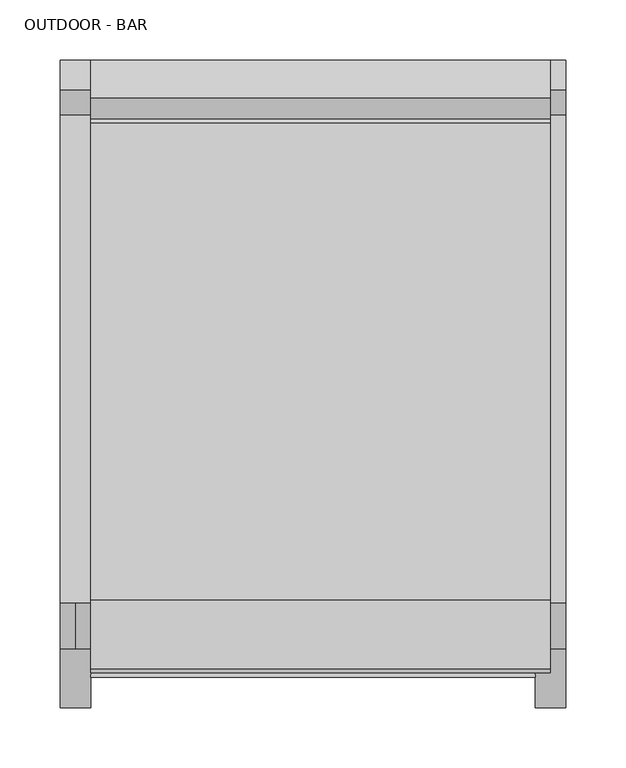
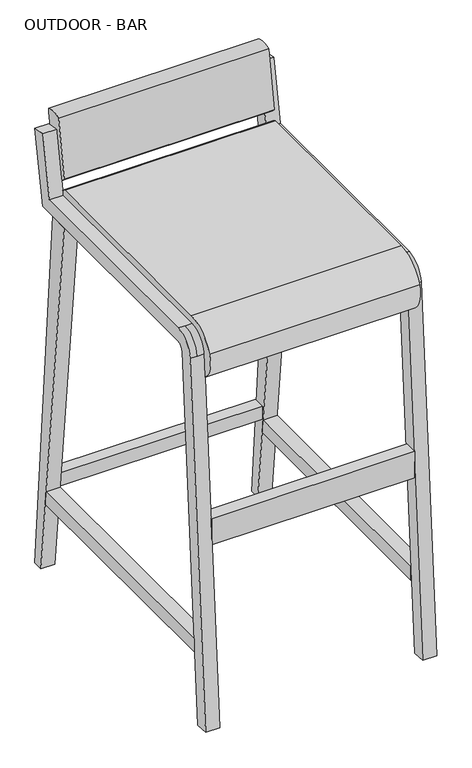
"""IFC4 building model written with IfcOpenShell, lengths in millimetres: furniture geometry, Bar_Stool_6722[1]1 : OUTDOOR - BAR."""

from ifc_helpers import new_model, si_unit, point, frame, frame_2d, origin, place, context, project, spatial, polyline, circle_curve, trimmed, segment, composite_curve, outline, extrude, source, transform, mapped, element, save
from ifc_brep_helpers import plane_surface, cylinder_surface, revolved_surface, advanced_brep


def outdoor_bar_9d95edac(model_context):
    return source(origin(), model_context, "Body", "SolidModel", [
        advanced_brep(
        [(419.1, -25.0141169, 838.4759165), (419.1, 0.0, 834.0652528), (393.7, 0.0, 834.0652528), (393.7, -25.0141169, 838.4759165), (393.7, -45.2169423, 723.9), (419.1, -45.2169423, 723.9), (393.7, -23.9038117, 698.5), (393.7, -450.0350637, 698.5), (393.7, -462.7032819, 686.6979128), (393.7, -511.439502, -0.8979128), (393.7, -536.7759384, 0.8979128), (393.7, -488.0397183, 688.4937383), (393.7, -450.0350637, 723.9), (419.1, -23.9038117, 698.5), (419.1, -450.0350637, 723.9), (419.1, -488.0397183, 688.4937383), (419.1, -536.7759384, 0.8979128), (419.1, -511.439502, -0.8979128), (419.1, -462.7032819, 686.6979128), (419.1, -450.0350637, 698.5), (406.4, -450.0350637, 723.9), (406.4, -488.0397183, 688.4937383)],
        [
            (0, 1),
            (1, 2),
            (2, 3),
            (3, 0),
            (3, 4),
            (4, 5),
            (5, 0),
            (2, 6),
            (6, 7),
            (7, 8, circle_curve(frame((393.7, -450.0350637, 685.8), z_axis=(1.0, 0.0, 0.0), x_axis=(0.0, 0.0, 1.0)), 12.7)),
            (8, 9),
            (9, 10),
            (10, 11),
            (11, 12, circle_curve(frame((393.7, -450.0350637, 685.8), z_axis=(-1.0, 0.0, 0.0), x_axis=(0.0, 0.0, 1.0)), 38.1)),
            (12, 4),
            (1, 13),
            (13, 6),
            (5, 14),
            (14, 15, circle_curve(frame((419.1, -450.0350637, 685.8), z_axis=(1.0, 0.0, 0.0), x_axis=(0.0, 0.0, 1.0)), 38.1)),
            (15, 16),
            (16, 17),
            (17, 18),
            (18, 19, circle_curve(frame((419.1, -450.0350637, 685.8), z_axis=(-1.0, 0.0, 0.0), x_axis=(0.0, 0.0, 1.0)), 12.7)),
            (19, 13),
            (12, 20),
            (20, 14),
            (19, 7),
            (21, 15),
            (20, 21, circle_curve(frame((406.4, -450.0350637, 685.8), z_axis=(1.0, 0.0, 0.0), x_axis=(0.0, 0.0, 1.0)), 38.1)),
            (11, 21),
            (18, 8),
            (10, 16),
            (17, 9),
        ],
        [
            plane_surface(frame((406.4, -12.5070585, 836.2705846), z_axis=(0.0, 0.17364817766692853, 0.9848077530122085), x_axis=(1.0, 0.0, 0.0))),
            plane_surface(frame((406.4, -25.0141169, 838.4759165), z_axis=(0.0, -0.9848077530122085, 0.17364817766692814), x_axis=(0.0, -0.17364817766692814, -0.9848077530122085))),
            plane_surface(frame((393.7, -25.0141169, 838.4759165), z_axis=(-1.0, 0.0, 0.0), x_axis=(0.0, -0.17364817766692808, -0.9848077530122085))),
            plane_surface(frame((393.7, 0.0, 834.0652528), z_axis=(0.0, 0.9848077530122085, -0.17364817766692817), x_axis=(0.0, -0.17364817766692817, -0.9848077530122085))),
            plane_surface(frame((419.1, 0.0, 834.0652528), z_axis=(1.0000000000000002, 0.0, 0.0), x_axis=(0.0, -0.1736481776669284, -0.9848077530122085))),
            plane_surface(frame((406.4, -45.2169423, 723.9), z_axis=(0.0, 0.0, 1.0), x_axis=(0.0, -1.0, 0.0))),
            plane_surface(frame((393.7, -23.9038117, 698.5), z_axis=(0.0, 0.0, -1.0), x_axis=(0.0, -1.0, 0.0))),
            cylinder_surface(frame((406.4, -450.0350637, 685.8), z_axis=(-1.0, 0.0, 0.0), x_axis=(0.0, 0.0, 1.0)), 38.1),
            revolved_surface(polyline([(393.7, -450.0350637, 698.5), (419.1, -450.0350637, 698.5)]), (406.4, -450.0350637, 685.8), (-1.0, 0.0, 0.0)),
            plane_surface(frame((406.4, -488.0397183, 688.4937383), z_axis=(0.0, -0.9974974969901172, 0.07070179275273744), x_axis=(0.0, -0.07070179275273744, -0.9974974969901172))),
            plane_surface(frame((393.7, -462.7032819, 686.6979128), z_axis=(0.0, 0.9974974969901172, -0.07070179275273743), x_axis=(0.0, -0.07070179275273743, -0.9974974969901172))),
            plane_surface(frame((406.4, -524.1077202, 0.0), z_axis=(0.0, -0.07070179275273399, -0.9974974969901175), x_axis=(1.0, 0.0, 0.0))),
        ],
        [
            (0, [[1, 2, 3, 4]]),
            (1, [[-4, 5, 6, 7]]),
            (2, [[8, 9, 10, 11, 12, 13, 14, 15, -5, -3]]),
            (3, [[16, 17, -8, -2]]),
            (4, [[-7, 18, 19, 20, 21, 22, 23, 24, -16, -1]]),
            (5, [[-15, 25, 26, -18, -6]]),
            (6, [[-24, 27, -9, -17]]),
            (7, [[28, -19, -26, 29]]),
            (7, [[30, -29, -25, -14]]),
            (8, [[31, -10, -27, -23]]),
            (9, [[32, -20, -28, -30, -13]]),
            (10, [[33, -11, -31, -22]]),
            (11, [[-12, -33, -21, -32]]),
        ],
    ),
        extrude(outline(composite_curve([segment(polyline([(-48.4096386, 756.5644068), (-31.5225381, 863.1853632)]), True, "CONTINUOUS"), segment(trimmed(circle_curve(frame_2d((-15.7612691, 828.3540875)), 38.2313401), [point((-31.5225381, 863.1853632))], [point((0.0, 863.1853632))], False, "CARTESIAN"), True, "CONTINUOUS"), segment(polyline([(0.0, 863.1853632), (0.0, 856.8353632), (-19.1416957, 748.2774126), (-44.0710693, 752.2258375), (-48.4096386, 756.5644068)]), True, "CONTINUOUS")], self_intersect=False)), frame((25.4, 0.0, 0.0), z_axis=(1.0, 0.0, 0.0), x_axis=(0.0, 1.0, 0.0)), (0.0, 0.0, 1.0), 381.0),
        extrude(outline(composite_curve([segment(polyline([(-51.6744261, 737.5144068), (-43.9498561, 733.0546243), (-46.417441, 704.85), (-452.817441, 704.85), (-460.5585493, 681.23302), (-460.5585493, 643.13302), (-484.2663236, 640.1699505)]), True, "CONTINUOUS"), segment(trimmed(circle_curve(frame_2d((-460.5585493, 681.23302)), 47.4155486), [point((-484.2663236, 640.1699505))], [point((-505.1145904, 697.4500928))], False, "CARTESIAN"), True, "CONTINUOUS"), segment(trimmed(circle_curve(frame_2d((-447.8968201, 676.6245275)), 60.8898793), [point((-505.1145904, 697.4500928))], [point((-447.8968201, 737.5144068))], False, "CARTESIAN"), True, "CONTINUOUS"), segment(polyline([(-447.8968201, 737.5144068), (-51.6744261, 737.5144068)]), True, "CONTINUOUS")], self_intersect=False)), frame((25.4, 0.0, 0.0), z_axis=(1.0, 0.0, 0.0), x_axis=(0.0, 1.0, 0.0)), (0.0, 0.0, 1.0), 381.0),
        extrude(outline(polyline([(393.7, -11.6871233), (393.7, -33.1441574), (25.4, -33.1441574), (25.4, -11.6871233), (393.7, -11.6871233)])), frame((0.0, 0.0, 157.9619127), z_axis=(0.0, 0.0, 1.0), x_axis=(1.0, 0.0, 0.0)), (0.0, 0.0, 1.0), 25.4),
        extrude(outline(polyline([(393.7, -488.2695397), (393.7, -511.439502), (25.4, -511.439502), (25.4, -488.2695397), (393.7, -488.2695397)])), frame((0.0, 0.0, 335.7619127), z_axis=(0.0, 0.0, 1.0), x_axis=(1.0, 0.0, 0.0)), (0.0, 0.0, 1.0), 50.8),
        extrude(outline(polyline([(-500.1796497, 157.9619127), (-35.652466, 157.9619127), (-32.9828185, 132.5619127), (-500.1796497, 132.5619127), (-500.1796497, 157.9619127)])), frame((393.7, 0.0, 0.0), z_axis=(1.0, 0.0, 0.0), x_axis=(0.0, 1.0, 0.0)), (0.0, 0.0, 1.0), 25.4),
        extrude(outline(polyline([(-500.1796497, 157.9619127), (-35.652466, 157.9619127), (-32.9828185, 132.5619127), (-500.1796497, 132.5619127), (-500.1796497, 157.9619127)])), frame((0.0, 0.0, 0.0), z_axis=(1.0, 0.0, 0.0), x_axis=(0.0, 1.0, 0.0)), (0.0, 0.0, 1.0), 25.4),
        extrude(outline(polyline([(0.0, 0.0), (-19.05, 0.0), (-92.4653083, 698.5), (-55.3031462, 698.5), (0.0, 0.0)])), frame((393.7, 0.0, 0.0), z_axis=(1.0, 0.0, 0.0), x_axis=(0.0, 1.0, 0.0)), (0.0, 0.0, 1.0), 25.4),
        advanced_brep(
        [(25.4, -25.0141169, 838.4759165), (25.4, 0.0, 834.0652528), (0.0, 0.0, 834.0652528), (0.0, -25.0141169, 838.4759165), (0.0, -45.2169423, 723.9), (25.4, -45.2169423, 723.9), (0.0, -23.9038117, 698.5), (0.0, -450.0350637, 698.5), (0.0, -462.7032819, 686.6979128), (0.0, -511.439502, -0.8979128), (0.0, -536.7759384, 0.8979128), (0.0, -488.0397183, 688.4937383), (0.0, -450.0350637, 723.9), (25.4, -23.9038117, 698.5), (25.4, -450.0350637, 723.9), (25.4, -488.0397183, 688.4937383), (25.4, -536.7759384, 0.8979128), (25.4, -511.439502, -0.8979128), (25.4, -462.7032819, 686.6979128), (25.4, -450.0350637, 698.5), (12.7, -450.0350637, 723.9), (12.7, -488.0397183, 688.4937383)],
        [
            (0, 1),
            (1, 2),
            (2, 3),
            (3, 0),
            (3, 4),
            (4, 5),
            (5, 0),
            (2, 6),
            (6, 7),
            (7, 8, circle_curve(frame((0.0, -450.0350637, 685.8), z_axis=(1.0, 0.0, 0.0), x_axis=(0.0, 0.0, 1.0)), 12.7)),
            (8, 9),
            (9, 10),
            (10, 11),
            (11, 12, circle_curve(frame((0.0, -450.0350637, 685.8), z_axis=(-1.0, 0.0, 0.0), x_axis=(0.0, 0.0, 1.0)), 38.1)),
            (12, 4),
            (1, 13),
            (13, 6),
            (5, 14),
            (14, 15, circle_curve(frame((25.4, -450.0350637, 685.8), z_axis=(1.0, 0.0, 0.0), x_axis=(0.0, 0.0, 1.0)), 38.1)),
            (15, 16),
            (16, 17),
            (17, 18),
            (18, 19, circle_curve(frame((25.4, -450.0350637, 685.8), z_axis=(-1.0, 0.0, 0.0), x_axis=(0.0, 0.0, 1.0)), 12.7)),
            (19, 13),
            (12, 20),
            (20, 14),
            (19, 7),
            (21, 15),
            (20, 21, circle_curve(frame((12.7, -450.0350637, 685.8), z_axis=(1.0, 0.0, 0.0), x_axis=(0.0, 0.0, 1.0)), 38.1)),
            (11, 21),
            (18, 8),
            (10, 16),
            (17, 9),
        ],
        [
            plane_surface(frame((12.7, -12.5070585, 836.2705846), z_axis=(0.0, 0.17364817766692853, 0.9848077530122085), x_axis=(1.0, 0.0, 0.0))),
            plane_surface(frame((12.7, -25.0141169, 838.4759165), z_axis=(0.0, -0.9848077530122085, 0.173648177666928), x_axis=(0.0, -0.173648177666928, -0.9848077530122085))),
            plane_surface(frame((0.0, -25.0141169, 838.4759165), z_axis=(-1.0, 0.0, 0.0), x_axis=(0.0, -0.17364817766692875, -0.9848077530122084))),
            plane_surface(frame((0.0, 0.0, 834.0652528), z_axis=(0.0, 0.9848077530122084, -0.17364817766692883), x_axis=(0.0, -0.17364817766692883, -0.9848077530122084))),
            plane_surface(frame((25.4, 0.0, 834.0652528), z_axis=(1.0000000000000002, 0.0, 0.0), x_axis=(0.0, -0.1736481776669284, -0.9848077530122085))),
            plane_surface(frame((12.7, -45.2169423, 723.9), z_axis=(0.0, 0.0, 1.0), x_axis=(0.0, -1.0, 0.0))),
            plane_surface(frame((0.0, -23.9038117, 698.5), z_axis=(0.0, 0.0, -1.0), x_axis=(0.0, -1.0, 0.0))),
            cylinder_surface(frame((12.7, -450.0350637, 685.8), z_axis=(-1.0, 0.0, 0.0), x_axis=(0.0, 0.0, 1.0)), 38.1),
            revolved_surface(polyline([(0.0, -450.0350637, 698.5), (25.4, -450.0350637, 698.5)]), (12.7, -450.0350637, 685.8), (-1.0, 0.0, 0.0)),
            plane_surface(frame((12.7, -488.0397183, 688.4937383), z_axis=(0.0, -0.9974974969901172, 0.07070179275273744), x_axis=(0.0, -0.07070179275273744, -0.9974974969901172))),
            plane_surface(frame((0.0, -462.7032819, 686.6979128), z_axis=(0.0, 0.9974974969901172, -0.07070179275273743), x_axis=(0.0, -0.07070179275273743, -0.9974974969901172))),
            plane_surface(frame((12.7, -524.1077202, 0.0), z_axis=(0.0, -0.07070179275273399, -0.9974974969901175), x_axis=(1.0, 0.0, 0.0))),
        ],
        [
            (0, [[1, 2, 3, 4]]),
            (1, [[-4, 5, 6, 7]]),
            (2, [[8, 9, 10, 11, 12, 13, 14, 15, -5, -3]]),
            (3, [[16, 17, -8, -2]]),
            (4, [[-7, 18, 19, 20, 21, 22, 23, 24, -16, -1]]),
            (5, [[-15, 25, 26, -18, -6]]),
            (6, [[-24, 27, -9, -17]]),
            (7, [[28, -19, -26, 29]]),
            (7, [[30, -29, -25, -14]]),
            (8, [[31, -10, -27, -23]]),
            (9, [[32, -20, -28, -30, -13]]),
            (10, [[33, -11, -31, -22]]),
            (11, [[-12, -33, -21, -32]]),
        ],
    ),
        extrude(outline(polyline([(0.0, 0.0), (-19.05, 0.0), (-92.4653083, 698.5), (-55.3031462, 698.5), (0.0, 0.0)])), frame((0.0, 0.0, 0.0), z_axis=(1.0, 0.0, 0.0), x_axis=(0.0, 1.0, 0.0)), (0.0, 0.0, 1.0), 25.4),
    ])


if __name__ == "__main__":
    model = new_model("IFC4")
    model_context = context("Model", 3, world=origin())
    ifc_project = project(units=[si_unit("LENGTHUNIT", "METRE", prefix="MILLI")], contexts=[model_context])
    site = spatial("IfcSite", under=ifc_project)
    building = spatial("IfcBuilding", under=site)
    placement = place(None, origin())
    outdoor_bar_shape = outdoor_bar_9d95edac(model_context)
    element("IfcFurniture", 1, ObjectType="Bar_Stool_6722[1]1 : OUTDOOR - BAR", at=placement, inside=building, context=model_context, shape_type="MappedRepresentation", body=[
        mapped(outdoor_bar_shape, transform((0.0, 0.0, 0.0), x_axis=(1.0, 0.0, 0.0), y_axis=(0.0, 1.0, 0.0), z_axis=(0.0, 0.0, 1.0))),
    ])
    save(model, "model.ifc")

# Revit data of these elements
# Type "Bar_Stool_6722[1]1 : OUTDOOR - BAR"
#   Type Mark = "TYPE - OUTDOOR - BAR"
#   Seating Count = 1
#   Seat = fab
#   Chair Legs = MET
# Element 1 (IfcFurniture, "Bar_Stool_6722[1]1 : OUTDOOR - BAR")
#   Materials on its faces: "MET", "fab"
# Materials
#   "fab": class "Leather", colour RGB 255 255 255, transparency 0, Cost = 0
#   "MET": class "Metal", colour RGB 189 187 185, transparency 0
